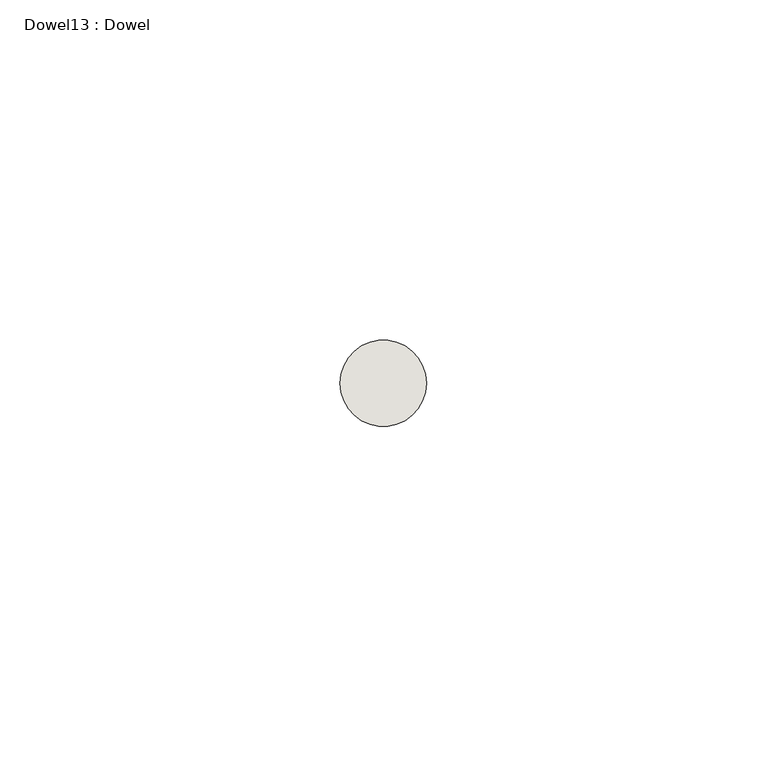
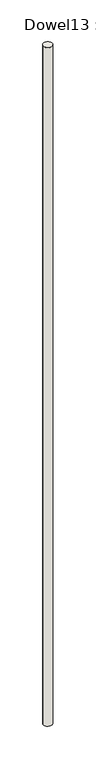
"""IFC4 building model written with IfcOpenShell, lengths in millimetres: wall geometry, Dowel13 : Dowel."""

from ifc_helpers import new_model, si_unit, point, frame, frame_2d, origin, place, context, project, spatial, circle_curve, trimmed, segment, composite_curve, outline, extrude, source, transform, mapped, element, save


def dowel13_dowel_3f6382b9(model_context):
    return source(origin(), model_context, "Body", "SweptSolid", [
        extrude(outline(composite_curve([segment(trimmed(circle_curve(frame_2d((373519.5134034, 446.88125)), 6.35), [point((373513.1634034, 446.88125))], [point((373525.8634034, 446.88125))], False, "CARTESIAN"), True, "CONTINUOUS"), segment(trimmed(circle_curve(frame_2d((373519.5134034, 446.88125)), 6.35), [point((373525.8634034, 446.88125))], [point((373513.1634034, 446.88125))], False, "CARTESIAN"), True, "CONTINUOUS")], self_intersect=False)), frame((0.0, 0.0, 1829.4958143), z_axis=(0.0, 0.0, 1.0), x_axis=(1.0, 0.0, 0.0)), (0.0, 0.0, 1.0), 1016.0),
    ])


if __name__ == "__main__":
    model = new_model("IFC4")
    model_context = context("Model", 3, world=origin())
    ifc_project = project(units=[si_unit("LENGTHUNIT", "METRE", prefix="MILLI")], contexts=[model_context])
    site = spatial("IfcSite", under=ifc_project)
    building = spatial("IfcBuilding", under=site)
    placement = place(None, origin())
    dowel13_dowel_shape = dowel13_dowel_3f6382b9(model_context)
    element("IfcWall", 1, ObjectType="Dowel13 : Dowel", at=placement, inside=building, context=model_context, shape_type="MappedRepresentation", body=[
        mapped(dowel13_dowel_shape, transform((0.0, 0.0, 0.0), x_axis=(1.0, 0.0, 0.0), y_axis=(0.0, 1.0, 0.0), z_axis=(0.0, 0.0, 1.0))),
    ])
    save(model, "model.ifc")

# Revit data of these elements
# Element 1 (IfcWall, "Dowel13 : Dowel")
#   Materials on its faces: "WALL REINFORCING - SEE PLAN SCHEDULES FOR SIZE/LOCATION"
# Materials
#   "WALL REINFORCING - SEE PLAN SCHEDULES FOR SIZE/LOCATION": class "Metal", colour RGB 189 187 185, transparency 0, Description = "Structural steel 50ksi", Cost = 0
